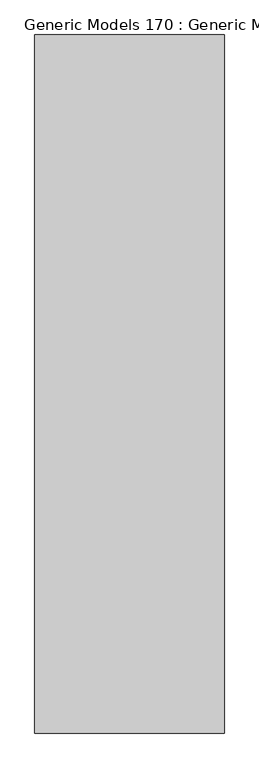
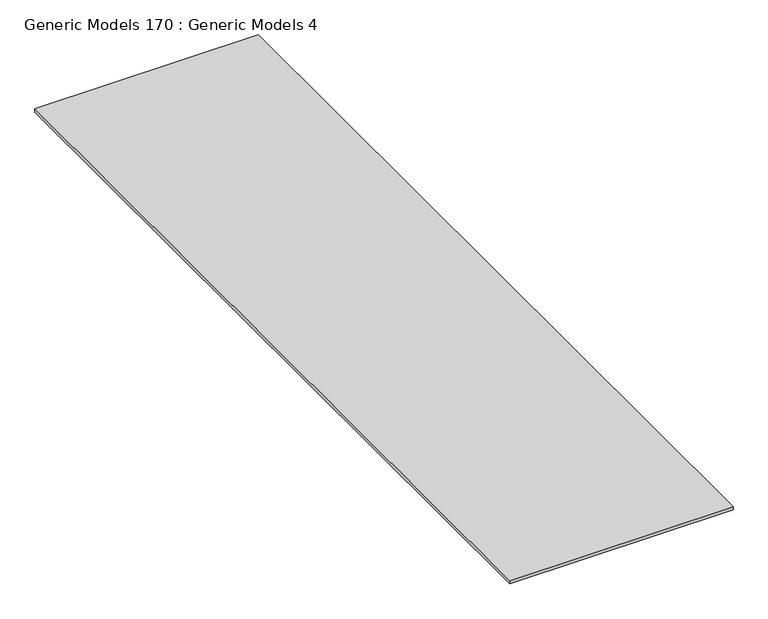
"""IFC4 building model written with IfcOpenShell, lengths in millimetres: proxy geometry, Generic Models 170 : Generic Models 4."""

from ifc_helpers import new_model, si_unit, frame, origin, place, context, project, spatial, polyline, outline, extrude, source, transform, mapped, element, save


def generic_models_170_generic_models_4_287c54e9(model_context):
    return source(origin(), model_context, "Body", "SweptSolid", [
        extrude(outline(polyline([(-6629.5736296, -5493.3230338), (-10037.6722239, -5493.3230338), (-10037.6722239, 7054.2769662), (-6629.5736296, 7054.2769662), (-6629.5736296, -5493.3230338)])), frame((0.0, 0.0, 122904.8484874), z_axis=(0.0, 0.0, 1.0), x_axis=(1.0, 0.0, 0.0)), (0.0, 0.0, 1.0), 50.8),
    ])


if __name__ == "__main__":
    model = new_model("IFC4")
    model_context = context("Model", 3, world=origin())
    ifc_project = project(units=[si_unit("LENGTHUNIT", "METRE", prefix="MILLI")], contexts=[model_context])
    site = spatial("IfcSite", under=ifc_project)
    building = spatial("IfcBuilding", under=site)
    placement = place(None, origin())
    generic_models_170_generic_models_4_shape = generic_models_170_generic_models_4_287c54e9(model_context)
    element("IfcBuildingElementProxy", 1, Name="Generic Models 170 : Generic Models 4", ObjectType="Generic Models 170 : Generic Models 4", at=placement, inside=building, context=model_context, shape_type="MappedRepresentation", body=[
        mapped(generic_models_170_generic_models_4_shape, transform((0.0, 0.0, 0.0), x_axis=(1.0, 0.0, 0.0), y_axis=(0.0, 1.0, 0.0), z_axis=(0.0, 0.0, 1.0))),
    ])
    save(model, "model.ifc")

# Revit data of these elements
# Element 1 (IfcBuildingElementProxy, "Generic Models 170 : Generic Models 4")
#   Materials on its faces: "_2\" SAND"
# Materials
#   "_2\" SAND": class "Generic", colour RGB 245 226 173, transparency 0, Cost = 0
